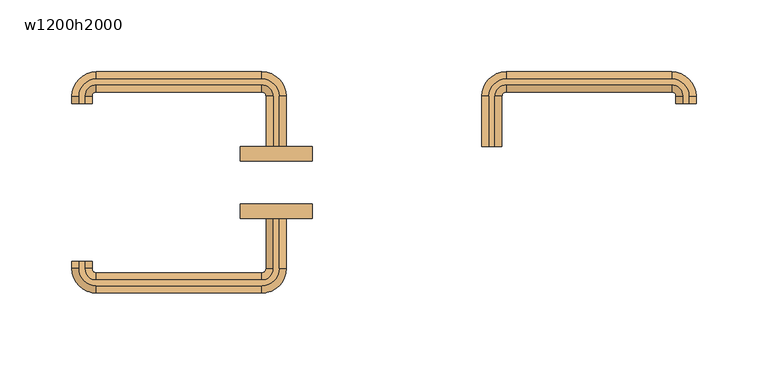
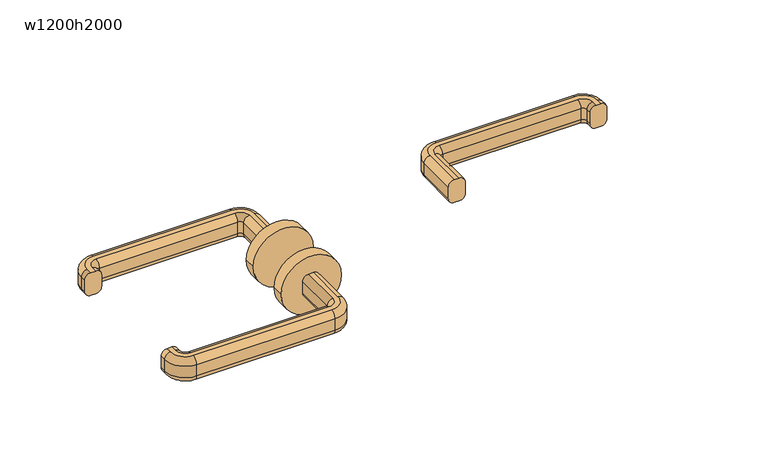
"""IFC4 building model written with IfcOpenShell, lengths in millimetres: door geometry, 二重 : w1200h2000."""

from ifc_helpers import new_model, si_unit, point, frame, frame_2d, origin, place, context, project, spatial, polyline, circle_curve, ellipse_curve, trimmed, segment, composite_curve, outline, extrude, source, transform, mapped, element, save
from ifc_brep_helpers import plane_surface, cylinder_surface, revolved_surface, advanced_brep


def w1200h2000_1489ebb8(model_context):
    return source(origin(), model_context, "Body", "SolidModel", [
        advanced_brep(
        [(-73.0, 95.0, 960.0), (-77.0, 95.0, 960.0), (-82.0, 95.0, 955.0), (-82.0, 95.0, 945.0477623), (-77.0, 95.0, 940.0477623), (-73.0, 95.0, 940.0477623), (-68.0, 95.0, 945.0477623), (-68.0, 95.0, 955.0), (-68.0, 130.0, 955.0), (-73.0, 130.0, 960.0), (-68.0, 130.0, 945.0477623), (-73.0, 130.0, 940.0477623), (-77.0, 130.0, 940.0477623), (-85.0, 138.0, 940.0477623), (-200.0, 138.0, 940.0477623), (-208.0, 130.0, 940.0477623), (-208.0, 125.0, 940.0477623), (-212.0, 125.0, 940.0477623), (-212.0, 130.0, 940.0477623), (-200.0, 142.0, 940.0477623), (-85.0, 142.0, 940.0477623), (-82.0, 130.0, 945.0477623), (-82.0, 130.0, 955.0), (-77.0, 130.0, 960.0), (-85.0, 142.0, 960.0), (-200.0, 142.0, 960.0), (-212.0, 130.0, 960.0), (-212.0, 125.0, 960.0), (-208.0, 125.0, 960.0), (-208.0, 130.0, 960.0), (-200.0, 138.0, 960.0), (-85.0, 138.0, 960.0), (-85.0, 147.0, 955.0), (-85.0, 147.0, 945.0477623), (-85.0, 133.0, 945.0477623), (-85.0, 133.0, 955.0), (-200.0, 147.0, 955.0), (-200.0, 147.0, 945.0477623), (-200.0, 133.0, 945.0477623), (-200.0, 133.0, 955.0), (-217.0, 130.0, 955.0), (-217.0, 130.0, 945.0477623), (-203.0, 130.0, 945.0477623), (-203.0, 130.0, 955.0), (-217.0, 125.0, 955.0), (-217.0, 125.0, 945.0477623), (-203.0, 125.0, 945.0477623), (-203.0, 125.0, 955.0)],
        [
            (0, 1),
            (1, 2, circle_curve(frame((-77.0, 95.0, 955.0), z_axis=(0.0, -1.0, 0.0), x_axis=(1.0, 0.0, 0.0)), 5.0)),
            (2, 3),
            (3, 4, circle_curve(frame((-77.0, 95.0, 945.0477623), z_axis=(0.0, -1.0, 0.0), x_axis=(1.0, 0.0, 0.0)), 5.0)),
            (4, 5),
            (5, 6, circle_curve(frame((-73.0, 95.0, 945.0477623), z_axis=(0.0, -1.0, 0.0), x_axis=(1.0, 0.0, 0.0)), 5.0)),
            (6, 7),
            (7, 0, circle_curve(frame((-73.0, 95.0, 955.0), z_axis=(0.0, -1.0, 0.0), x_axis=(1.0, 0.0, 0.0)), 5.0)),
            (7, 8),
            (8, 9, circle_curve(frame((-73.0, 130.0, 955.0), z_axis=(0.0, -1.0, 0.0), x_axis=(1.0, 0.0, 0.0)), 5.0)),
            (9, 0),
            (6, 10),
            (10, 8),
            (5, 11),
            (11, 10, circle_curve(frame((-73.0, 130.0, 945.0477623), z_axis=(0.0, -1.0, 0.0), x_axis=(1.0, 0.0, 0.0)), 5.0)),
            (4, 12),
            (12, 13, circle_curve(frame((-85.0, 130.0, 940.0477623), z_axis=(0.0, 0.0, 1.0), x_axis=(1.0, 0.0, 0.0)), 8.0)),
            (13, 14),
            (14, 15, circle_curve(frame((-200.0, 130.0, 940.0477623), z_axis=(0.0, 0.0, 1.0), x_axis=(0.0, 1.0, 0.0)), 8.0)),
            (15, 16),
            (16, 17),
            (17, 18),
            (18, 19, circle_curve(frame((-200.0, 130.0, 940.0477623), z_axis=(0.0, 0.0, -1.0), x_axis=(0.0, 1.0, 0.0)), 12.0)),
            (19, 20),
            (20, 11, circle_curve(frame((-85.0, 130.0, 940.0477623), z_axis=(0.0, 0.0, -1.0), x_axis=(1.0, 0.0, 0.0)), 12.0)),
            (3, 21),
            (21, 12, circle_curve(frame((-77.0, 130.0, 945.0477623), z_axis=(0.0, -1.0, 0.0), x_axis=(1.0, 0.0, 0.0)), 5.0)),
            (2, 22),
            (22, 21),
            (1, 23),
            (23, 22, circle_curve(frame((-77.0, 130.0, 955.0), z_axis=(0.0, -1.0, 0.0), x_axis=(1.0, 0.0, 0.0)), 5.0)),
            (9, 24, circle_curve(frame((-85.0, 130.0, 960.0), z_axis=(0.0, 0.0, 1.0), x_axis=(1.0, 0.0, 0.0)), 12.0)),
            (24, 25),
            (25, 26, circle_curve(frame((-200.0, 130.0, 960.0), z_axis=(0.0, 0.0, 1.0), x_axis=(0.0, 1.0, 0.0)), 12.0)),
            (26, 27),
            (27, 28),
            (28, 29),
            (29, 30, circle_curve(frame((-200.0, 130.0, 960.0), z_axis=(0.0, 0.0, -1.0), x_axis=(0.0, 1.0, 0.0)), 8.0)),
            (30, 31),
            (31, 23, circle_curve(frame((-85.0, 130.0, 960.0), z_axis=(0.0, 0.0, -1.0), x_axis=(1.0, 0.0, 0.0)), 8.0)),
            (32, 24, circle_curve(frame((-85.0, 142.0, 955.0), z_axis=(1.0, 0.0, 0.0), x_axis=(0.0, 1.0, 0.0)), 5.0)),
            (8, 32, circle_curve(frame((-85.0, 130.0, 955.0), z_axis=(0.0, 0.0, 1.0), x_axis=(1.0, 0.0, 0.0)), 17.0)),
            (33, 32),
            (10, 33, circle_curve(frame((-85.0, 130.0, 945.0477623), z_axis=(0.0, 0.0, 1.0), x_axis=(1.0, 0.0, 0.0)), 17.0)),
            (20, 33, circle_curve(frame((-85.0, 142.0, 945.0477623), z_axis=(1.0, 0.0, 0.0), x_axis=(0.0, 1.0, 0.0)), 5.0)),
            (34, 13, circle_curve(frame((-85.0, 138.0, 945.0477623), z_axis=(1.0, 0.0, 0.0), x_axis=(0.0, 1.0, 0.0)), 5.0)),
            (21, 34, circle_curve(frame((-85.0, 130.0, 945.0477623), z_axis=(0.0, 0.0, 1.0), x_axis=(1.0, 0.0, 0.0)), 3.0)),
            (35, 34),
            (22, 35, circle_curve(frame((-85.0, 130.0, 955.0), z_axis=(0.0, 0.0, 1.0), x_axis=(1.0, 0.0, 0.0)), 3.0)),
            (31, 35, circle_curve(frame((-85.0, 138.0, 955.0), z_axis=(1.0, 0.0, 0.0), x_axis=(0.0, 1.0, 0.0)), 5.0)),
            (32, 36),
            (36, 25, circle_curve(frame((-200.0, 142.0, 955.0), z_axis=(1.0, 0.0, 0.0), x_axis=(0.0, 1.0, 0.0)), 5.0)),
            (33, 37),
            (37, 36),
            (19, 37, circle_curve(frame((-200.0, 142.0, 945.0477623), z_axis=(1.0, 0.0, 0.0), x_axis=(0.0, 1.0, 0.0)), 5.0)),
            (34, 38),
            (38, 14, circle_curve(frame((-200.0, 138.0, 945.0477623), z_axis=(1.0, 0.0, 0.0), x_axis=(0.0, 1.0, 0.0)), 5.0)),
            (35, 39),
            (39, 38),
            (30, 39, circle_curve(frame((-200.0, 138.0, 955.0), z_axis=(1.0, 0.0, 0.0), x_axis=(0.0, 1.0, 0.0)), 5.0)),
            (40, 26, circle_curve(frame((-212.0, 130.0, 955.0), z_axis=(0.0, 1.0, 0.0), x_axis=(-1.0, 0.0, 0.0)), 5.0)),
            (36, 40, circle_curve(frame((-200.0, 130.0, 955.0), z_axis=(0.0, 0.0, 1.0), x_axis=(0.0, 1.0, 0.0)), 17.0)),
            (41, 40),
            (37, 41, circle_curve(frame((-200.0, 130.0, 945.0477623), z_axis=(0.0, 0.0, 1.0), x_axis=(0.0, 1.0, 0.0)), 17.0)),
            (18, 41, circle_curve(frame((-212.0, 130.0, 945.0477623), z_axis=(0.0, 1.0, 0.0), x_axis=(-1.0, 0.0, 0.0)), 5.0)),
            (42, 15, circle_curve(frame((-208.0, 130.0, 945.0477623), z_axis=(0.0, 1.0, 0.0), x_axis=(-1.0, 0.0, 0.0)), 5.0)),
            (38, 42, circle_curve(frame((-200.0, 130.0, 945.0477623), z_axis=(0.0, 0.0, 1.0), x_axis=(0.0, 1.0, 0.0)), 3.0)),
            (43, 42),
            (39, 43, circle_curve(frame((-200.0, 130.0, 955.0), z_axis=(0.0, 0.0, 1.0), x_axis=(0.0, 1.0, 0.0)), 3.0)),
            (29, 43, circle_curve(frame((-208.0, 130.0, 955.0), z_axis=(0.0, 1.0, 0.0), x_axis=(-1.0, 0.0, 0.0)), 5.0)),
            (27, 44, circle_curve(frame((-212.0, 125.0, 955.0), z_axis=(0.0, -1.0, 0.0), x_axis=(-1.0, 0.0, 0.0)), 5.0)),
            (44, 45),
            (45, 17, circle_curve(frame((-212.0, 125.0, 945.0477623), z_axis=(0.0, -1.0, 0.0), x_axis=(-1.0, 0.0, 0.0)), 5.0)),
            (16, 46, circle_curve(frame((-208.0, 125.0, 945.0477623), z_axis=(0.0, -1.0, 0.0), x_axis=(-1.0, 0.0, 0.0)), 5.0)),
            (46, 47),
            (47, 28, circle_curve(frame((-208.0, 125.0, 955.0), z_axis=(0.0, -1.0, 0.0), x_axis=(-1.0, 0.0, 0.0)), 5.0)),
            (40, 44),
            (41, 45),
            (42, 46),
            (43, 47),
        ],
        [
            plane_surface(frame((-64.801961, 95.0, 950.0), z_axis=(0.0, -1.0, 0.0), x_axis=(0.0, 0.0, 1.0))),
            cylinder_surface(frame((-73.0, 95.0, 955.0), z_axis=(0.0, -1.0, 0.0), x_axis=(1.0, 0.0, 0.0)), 5.0),
            plane_surface(frame((-68.0, 95.0, 955.0), z_axis=(1.0, 0.0, 0.0), x_axis=(0.0, 1.0, 0.0))),
            cylinder_surface(frame((-73.0, 95.0, 945.0477623), z_axis=(0.0, -1.0, 0.0), x_axis=(1.0, 0.0, 0.0)), 5.0),
            plane_surface(frame((-73.0, 95.0, 940.0477623), z_axis=(0.0, 0.0, -1.0), x_axis=(0.0, 1.0, 0.0))),
            cylinder_surface(frame((-77.0, 95.0, 945.0477623), z_axis=(0.0, -1.0, 0.0), x_axis=(1.0, 0.0, 0.0)), 5.0),
            plane_surface(frame((-82.0, 95.0, 945.0477623), z_axis=(-1.0, 0.0, 0.0), x_axis=(0.0, 1.0, 0.0))),
            cylinder_surface(frame((-77.0, 95.0, 955.0), z_axis=(0.0, -1.0, 0.0), x_axis=(1.0, 0.0, 0.0)), 5.0),
            plane_surface(frame((-77.0, 95.0, 960.0), z_axis=(0.0, 0.0, 1.0), x_axis=(0.0, 1.0, 0.0))),
            revolved_surface(trimmed(ellipse_curve(frame((-73.0, 130.0, 955.0), z_axis=(0.0, 1.0, 0.0), x_axis=(1.0, 0.0, 0.0)), 5.0, 5.0), [point((-73.0, 130.0, 960.0))], [point((-68.0, 130.0, 955.0))], True, "CARTESIAN"), (-85.0, 130.0, 950.0), (0.0, 0.0, -1.0)),
            cylinder_surface(frame((-85.0, 130.0, 950.0), z_axis=(0.0, 0.0, -1.0), x_axis=(1.0, 0.0, 0.0)), 17.0),
            revolved_surface(trimmed(ellipse_curve(frame((-73.0, 130.0, 945.0477623), z_axis=(0.0, 1.0, 0.0), x_axis=(1.0, 0.0, 0.0)), 5.0, 5.0), [point((-68.0, 130.0, 945.0477623))], [point((-73.0, 130.0, 940.0477623))], True, "CARTESIAN"), (-85.0, 130.0, 950.0), (0.0, 0.0, -1.0)),
            revolved_surface(trimmed(ellipse_curve(frame((-77.0, 130.0, 945.0477623), z_axis=(0.0, 1.0, 0.0), x_axis=(1.0, 0.0, 0.0)), 5.0, 5.0), [point((-77.0, 130.0, 940.0477623))], [point((-82.0, 130.0, 945.0477623))], True, "CARTESIAN"), (-85.0, 130.0, 950.0), (0.0, 0.0, -1.0)),
            revolved_surface(polyline([(-82.0, 130.0, 945.0477623), (-82.0, 130.0, 955.0)]), (-85.0, 130.0, 950.0), (0.0, 0.0, -1.0)),
            revolved_surface(trimmed(ellipse_curve(frame((-77.0, 130.0, 955.0), z_axis=(0.0, 1.0, 0.0), x_axis=(1.0, 0.0, 0.0)), 5.0, 5.0), [point((-82.0, 130.0, 955.0))], [point((-77.0, 130.0, 960.0))], True, "CARTESIAN"), (-85.0, 130.0, 950.0), (0.0, 0.0, -1.0)),
            cylinder_surface(frame((-85.0, 142.0, 955.0), z_axis=(1.0, 0.0, 0.0), x_axis=(0.0, 1.0, 0.0)), 5.0),
            plane_surface(frame((-85.0, 147.0, 955.0), z_axis=(0.0, 1.0, 0.0), x_axis=(-1.0, 0.0, 0.0))),
            cylinder_surface(frame((-85.0, 142.0, 945.0477623), z_axis=(1.0, 0.0, 0.0), x_axis=(0.0, 1.0, 0.0)), 5.0),
            cylinder_surface(frame((-85.0, 138.0, 945.0477623), z_axis=(1.0, 0.0, 0.0), x_axis=(0.0, 1.0, 0.0)), 5.0),
            plane_surface(frame((-85.0, 133.0, 945.0477623), z_axis=(0.0, -1.0, 0.0), x_axis=(-1.0, 0.0, 0.0))),
            cylinder_surface(frame((-85.0, 138.0, 955.0), z_axis=(1.0, 0.0, 0.0), x_axis=(0.0, 1.0, 0.0)), 5.0),
            revolved_surface(trimmed(ellipse_curve(frame((-200.0, 142.0, 955.0), z_axis=(-1.0, 0.0, 0.0), x_axis=(0.0, 1.0, 0.0)), 5.0, 5.0), [point((-200.0, 142.0, 960.0))], [point((-200.0, 147.0, 955.0))], True, "CARTESIAN"), (-200.0, 130.0, 950.0), (0.0, 0.0, -1.0)),
            cylinder_surface(frame((-200.0, 130.0, 950.0), z_axis=(0.0, 0.0, -1.0), x_axis=(0.0, 1.0, 0.0)), 17.0),
            revolved_surface(trimmed(ellipse_curve(frame((-200.0, 142.0, 945.0477623), z_axis=(-1.0, 0.0, 0.0), x_axis=(0.0, 1.0, 0.0)), 5.0, 5.0), [point((-200.0, 147.0, 945.0477623))], [point((-200.0, 142.0, 940.0477623))], True, "CARTESIAN"), (-200.0, 130.0, 950.0), (0.0, 0.0, -1.0)),
            revolved_surface(trimmed(ellipse_curve(frame((-200.0, 138.0, 945.0477623), z_axis=(-1.0, 0.0, 0.0), x_axis=(0.0, 1.0, 0.0)), 5.0, 5.0), [point((-200.0, 138.0, 940.0477623))], [point((-200.0, 133.0, 945.0477623))], True, "CARTESIAN"), (-200.0, 130.0, 950.0), (0.0, 0.0, -1.0)),
            revolved_surface(polyline([(-200.0, 133.0, 945.0477623), (-200.0, 133.0, 955.0)]), (-200.0, 130.0, 950.0), (0.0, 0.0, -1.0)),
            revolved_surface(trimmed(ellipse_curve(frame((-200.0, 138.0, 955.0), z_axis=(-1.0, 0.0, 0.0), x_axis=(0.0, 1.0, 0.0)), 5.0, 5.0), [point((-200.0, 133.0, 955.0))], [point((-200.0, 138.0, 960.0))], True, "CARTESIAN"), (-200.0, 130.0, 950.0), (0.0, 0.0, -1.0)),
            plane_surface(frame((-199.801961, 125.0, 950.0), z_axis=(0.0, -1.0, 0.0), x_axis=(0.0, 0.0, -1.0))),
            cylinder_surface(frame((-212.0, 130.0, 955.0), z_axis=(0.0, 1.0, 0.0), x_axis=(-1.0, 0.0, 0.0)), 5.0),
            plane_surface(frame((-217.0, 130.0, 955.0), z_axis=(-1.0, 0.0, 0.0), x_axis=(0.0, -1.0, 0.0))),
            cylinder_surface(frame((-212.0, 130.0, 945.0477623), z_axis=(0.0, 1.0, 0.0), x_axis=(-1.0, 0.0, 0.0)), 5.0),
            cylinder_surface(frame((-208.0, 130.0, 945.0477623), z_axis=(0.0, 1.0, 0.0), x_axis=(-1.0, 0.0, 0.0)), 5.0),
            plane_surface(frame((-203.0, 130.0, 945.0477623), z_axis=(1.0, 0.0, 0.0), x_axis=(0.0, -1.0, 0.0))),
            cylinder_surface(frame((-208.0, 130.0, 955.0), z_axis=(0.0, 1.0, 0.0), x_axis=(-1.0, 0.0, 0.0)), 5.0),
        ],
        [
            (0, [[1, 2, 3, 4, 5, 6, 7, 8]]),
            (1, [[9, 10, 11, -8]]),
            (2, [[12, 13, -9, -7]]),
            (3, [[14, 15, -12, -6]]),
            (4, [[16, 17, 18, 19, 20, 21, 22, 23, 24, 25, -14, -5]]),
            (5, [[26, 27, -16, -4]]),
            (6, [[28, 29, -26, -3]]),
            (7, [[30, 31, -28, -2]]),
            (8, [[-11, 32, 33, 34, 35, 36, 37, 38, 39, 40, -30, -1]]),
            (9, [[41, -32, -10, 42]]),
            (10, [[43, -42, -13, 44]]),
            (11, [[45, -44, -15, -25]]),
            (12, [[46, -17, -27, 47]]),
            (13, [[48, -47, -29, 49]]),
            (14, [[50, -49, -31, -40]]),
            (15, [[51, 52, -33, -41]]),
            (16, [[53, 54, -51, -43]]),
            (17, [[-24, 55, -53, -45]]),
            (18, [[56, 57, -18, -46]]),
            (19, [[58, 59, -56, -48]]),
            (20, [[-39, 60, -58, -50]]),
            (21, [[61, -34, -52, 62]]),
            (22, [[63, -62, -54, 64]]),
            (23, [[65, -64, -55, -23]]),
            (24, [[66, -19, -57, 67]]),
            (25, [[68, -67, -59, 69]]),
            (26, [[70, -69, -60, -38]]),
            (27, [[71, 72, 73, -21, 74, 75, 76, -36]]),
            (28, [[77, -71, -35, -61]]),
            (29, [[78, -72, -77, -63]]),
            (30, [[-22, -73, -78, -65]]),
            (31, [[79, -74, -20, -66]]),
            (32, [[80, -75, -79, -68]]),
            (33, [[-37, -76, -80, -70]]),
        ],
    ),
        advanced_brep(
        [(-77.0, 45.0, 940.0), (-82.0, 45.0, 945.0), (-82.0, 45.0, 955.0), (-77.0, 45.0, 960.0), (-73.0, 45.0, 960.0), (-68.0, 45.0, 955.0), (-68.0, 45.0, 945.0), (-73.0, 45.0, 940.0), (-73.0, 10.0, 940.0), (-85.0, -2.0, 940.0), (-200.0, -2.0, 940.0), (-212.0, 10.0, 940.0), (-212.0, 15.0, 940.0), (-208.0, 15.0, 940.0), (-208.0, 10.0, 940.0), (-200.0, 2.0, 940.0), (-85.0, 2.0, 940.0), (-77.0, 10.0, 940.0), (-68.0, 10.0, 945.0), (-68.0, 10.0, 955.0), (-73.0, 10.0, 960.0), (-77.0, 10.0, 960.0), (-85.0, 2.0, 960.0), (-200.0, 2.0, 960.0), (-208.0, 10.0, 960.0), (-208.0, 15.0, 960.0), (-212.0, 15.0, 960.0), (-212.0, 10.0, 960.0), (-200.0, -2.0, 960.0), (-85.0, -2.0, 960.0), (-82.0, 10.0, 955.0), (-82.0, 10.0, 945.0), (-85.0, -7.0, 945.0), (-85.0, -7.0, 955.0), (-85.0, 7.0, 955.0), (-85.0, 7.0, 945.0), (-200.0, -7.0, 945.0), (-200.0, -7.0, 955.0), (-200.0, 7.0, 955.0), (-200.0, 7.0, 945.0), (-217.0, 10.0, 945.0), (-217.0, 10.0, 955.0), (-203.0, 10.0, 955.0), (-203.0, 10.0, 945.0), (-217.0, 15.0, 945.0), (-217.0, 15.0, 955.0), (-203.0, 15.0, 955.0), (-203.0, 15.0, 945.0)],
        [
            (0, 1, circle_curve(frame((-77.0, 45.0, 945.0), z_axis=(0.0, 1.0, 0.0), x_axis=(-1.0, 0.0, 0.0)), 5.0)),
            (1, 2),
            (2, 3, circle_curve(frame((-77.0, 45.0, 955.0), z_axis=(0.0, 1.0, 0.0), x_axis=(-1.0, 0.0, 0.0)), 5.0)),
            (3, 4),
            (4, 5, circle_curve(frame((-73.0, 45.0, 955.0), z_axis=(0.0, 1.0, 0.0), x_axis=(-1.0, 0.0, 0.0)), 5.0)),
            (5, 6),
            (6, 7, circle_curve(frame((-73.0, 45.0, 945.0), z_axis=(0.0, 1.0, 0.0), x_axis=(-1.0, 0.0, 0.0)), 5.0)),
            (7, 0),
            (7, 8),
            (8, 9, circle_curve(frame((-85.0, 10.0, 940.0), z_axis=(0.0, 0.0, -1.0), x_axis=(1.0, 0.0, 0.0)), 12.0)),
            (9, 10),
            (10, 11, circle_curve(frame((-200.0, 10.0, 940.0), z_axis=(0.0, 0.0, -1.0), x_axis=(0.0, -1.0, 0.0)), 12.0)),
            (11, 12),
            (12, 13),
            (13, 14),
            (14, 15, circle_curve(frame((-200.0, 10.0, 940.0), z_axis=(0.0, 0.0, 1.0), x_axis=(0.0, -1.0, 0.0)), 8.0)),
            (15, 16),
            (16, 17, circle_curve(frame((-85.0, 10.0, 940.0), z_axis=(0.0, 0.0, 1.0), x_axis=(1.0, 0.0, 0.0)), 8.0)),
            (17, 0),
            (6, 18),
            (18, 8, circle_curve(frame((-73.0, 10.0, 945.0), z_axis=(0.0, 1.0, 0.0), x_axis=(-1.0, 0.0, 0.0)), 5.0)),
            (5, 19),
            (19, 18),
            (4, 20),
            (20, 19, circle_curve(frame((-73.0, 10.0, 955.0), z_axis=(0.0, 1.0, 0.0), x_axis=(-1.0, 0.0, 0.0)), 5.0)),
            (3, 21),
            (21, 22, circle_curve(frame((-85.0, 10.0, 960.0), z_axis=(0.0, 0.0, -1.0), x_axis=(1.0, 0.0, 0.0)), 8.0)),
            (22, 23),
            (23, 24, circle_curve(frame((-200.0, 10.0, 960.0), z_axis=(0.0, 0.0, -1.0), x_axis=(0.0, -1.0, 0.0)), 8.0)),
            (24, 25),
            (25, 26),
            (26, 27),
            (27, 28, circle_curve(frame((-200.0, 10.0, 960.0), z_axis=(0.0, 0.0, 1.0), x_axis=(0.0, -1.0, 0.0)), 12.0)),
            (28, 29),
            (29, 20, circle_curve(frame((-85.0, 10.0, 960.0), z_axis=(0.0, 0.0, 1.0), x_axis=(1.0, 0.0, 0.0)), 12.0)),
            (2, 30),
            (30, 21, circle_curve(frame((-77.0, 10.0, 955.0), z_axis=(0.0, 1.0, 0.0), x_axis=(-1.0, 0.0, 0.0)), 5.0)),
            (1, 31),
            (31, 30),
            (17, 31, circle_curve(frame((-77.0, 10.0, 945.0), z_axis=(0.0, 1.0, 0.0), x_axis=(-1.0, 0.0, 0.0)), 5.0)),
            (32, 9, circle_curve(frame((-85.0, -2.0, 945.0), z_axis=(1.0, 0.0, 0.0), x_axis=(0.0, 1.0, 0.0)), 5.0)),
            (18, 32, circle_curve(frame((-85.0, 10.0, 945.0), z_axis=(0.0, 0.0, -1.0), x_axis=(1.0, 0.0, 0.0)), 17.0)),
            (33, 32),
            (19, 33, circle_curve(frame((-85.0, 10.0, 955.0), z_axis=(0.0, 0.0, -1.0), x_axis=(1.0, 0.0, 0.0)), 17.0)),
            (29, 33, circle_curve(frame((-85.0, -2.0, 955.0), z_axis=(1.0, 0.0, 0.0), x_axis=(0.0, 1.0, 0.0)), 5.0)),
            (34, 22, circle_curve(frame((-85.0, 2.0, 955.0), z_axis=(1.0, 0.0, 0.0), x_axis=(0.0, 1.0, 0.0)), 5.0)),
            (30, 34, circle_curve(frame((-85.0, 10.0, 955.0), z_axis=(0.0, 0.0, -1.0), x_axis=(1.0, 0.0, 0.0)), 3.0)),
            (35, 34),
            (31, 35, circle_curve(frame((-85.0, 10.0, 945.0), z_axis=(0.0, 0.0, -1.0), x_axis=(1.0, 0.0, 0.0)), 3.0)),
            (16, 35, circle_curve(frame((-85.0, 2.0, 945.0), z_axis=(1.0, 0.0, 0.0), x_axis=(0.0, 1.0, 0.0)), 5.0)),
            (32, 36),
            (36, 10, circle_curve(frame((-200.0, -2.0, 945.0), z_axis=(1.0, 0.0, 0.0), x_axis=(0.0, 1.0, 0.0)), 5.0)),
            (33, 37),
            (37, 36),
            (28, 37, circle_curve(frame((-200.0, -2.0, 955.0), z_axis=(1.0, 0.0, 0.0), x_axis=(0.0, 1.0, 0.0)), 5.0)),
            (34, 38),
            (38, 23, circle_curve(frame((-200.0, 2.0, 955.0), z_axis=(1.0, 0.0, 0.0), x_axis=(0.0, 1.0, 0.0)), 5.0)),
            (35, 39),
            (39, 38),
            (15, 39, circle_curve(frame((-200.0, 2.0, 945.0), z_axis=(1.0, 0.0, 0.0), x_axis=(0.0, 1.0, 0.0)), 5.0)),
            (40, 11, circle_curve(frame((-212.0, 10.0, 945.0), z_axis=(0.0, -1.0, 0.0), x_axis=(1.0, 0.0, 0.0)), 5.0)),
            (36, 40, circle_curve(frame((-200.0, 10.0, 945.0), z_axis=(0.0, 0.0, -1.0), x_axis=(0.0, -1.0, 0.0)), 17.0)),
            (41, 40),
            (37, 41, circle_curve(frame((-200.0, 10.0, 955.0), z_axis=(0.0, 0.0, -1.0), x_axis=(0.0, -1.0, 0.0)), 17.0)),
            (27, 41, circle_curve(frame((-212.0, 10.0, 955.0), z_axis=(0.0, -1.0, 0.0), x_axis=(1.0, 0.0, 0.0)), 5.0)),
            (42, 24, circle_curve(frame((-208.0, 10.0, 955.0), z_axis=(0.0, -1.0, 0.0), x_axis=(1.0, 0.0, 0.0)), 5.0)),
            (38, 42, circle_curve(frame((-200.0, 10.0, 955.0), z_axis=(0.0, 0.0, -1.0), x_axis=(0.0, -1.0, 0.0)), 3.0)),
            (43, 42),
            (39, 43, circle_curve(frame((-200.0, 10.0, 945.0), z_axis=(0.0, 0.0, -1.0), x_axis=(0.0, -1.0, 0.0)), 3.0)),
            (14, 43, circle_curve(frame((-208.0, 10.0, 945.0), z_axis=(0.0, -1.0, 0.0), x_axis=(1.0, 0.0, 0.0)), 5.0)),
            (12, 44, circle_curve(frame((-212.0, 15.0, 945.0), z_axis=(0.0, 1.0, 0.0), x_axis=(1.0, 0.0, 0.0)), 5.0)),
            (44, 45),
            (45, 26, circle_curve(frame((-212.0, 15.0, 955.0), z_axis=(0.0, 1.0, 0.0), x_axis=(1.0, 0.0, 0.0)), 5.0)),
            (25, 46, circle_curve(frame((-208.0, 15.0, 955.0), z_axis=(0.0, 1.0, 0.0), x_axis=(1.0, 0.0, 0.0)), 5.0)),
            (46, 47),
            (47, 13, circle_curve(frame((-208.0, 15.0, 945.0), z_axis=(0.0, 1.0, 0.0), x_axis=(1.0, 0.0, 0.0)), 5.0)),
            (40, 44),
            (41, 45),
            (42, 46),
            (43, 47),
        ],
        [
            plane_surface(frame((-64.801961, 45.0, 950.0), z_axis=(0.0, 1.0, 0.0), x_axis=(0.0, 0.0, -1.0))),
            plane_surface(frame((-77.0, 45.0, 940.0), z_axis=(0.0, 0.0, -1.0), x_axis=(0.0, -1.0, 0.0))),
            cylinder_surface(frame((-73.0, 45.0, 945.0), z_axis=(0.0, 1.0, 0.0), x_axis=(-1.0, 0.0, 0.0)), 5.0),
            plane_surface(frame((-68.0, 45.0, 945.0), z_axis=(1.0, 0.0, 0.0), x_axis=(0.0, -1.0, 0.0))),
            cylinder_surface(frame((-73.0, 45.0, 955.0), z_axis=(0.0, 1.0, 0.0), x_axis=(-1.0, 0.0, 0.0)), 5.0),
            plane_surface(frame((-73.0, 45.0, 960.0), z_axis=(0.0, 0.0, 1.0), x_axis=(0.0, -1.0, 0.0))),
            cylinder_surface(frame((-77.0, 45.0, 955.0), z_axis=(0.0, 1.0, 0.0), x_axis=(-1.0, 0.0, 0.0)), 5.0),
            plane_surface(frame((-82.0, 45.0, 955.0), z_axis=(-1.0, 0.0, 0.0), x_axis=(0.0, -1.0, 0.0))),
            cylinder_surface(frame((-77.0, 45.0, 945.0), z_axis=(0.0, 1.0, 0.0), x_axis=(-1.0, 0.0, 0.0)), 5.0),
            revolved_surface(trimmed(ellipse_curve(frame((-73.0, 10.0, 945.0), z_axis=(0.0, -1.0, 0.0), x_axis=(-1.0, 0.0, 0.0)), 5.0, 5.0), [point((-73.0, 10.0, 940.0))], [point((-68.0, 10.0, 945.0))], True, "CARTESIAN"), (-85.0, 10.0, 950.0), (0.0, 0.0, 1.0)),
            cylinder_surface(frame((-85.0, 10.0, 950.0), z_axis=(0.0, 0.0, 1.0), x_axis=(1.0, 0.0, 0.0)), 17.0),
            revolved_surface(trimmed(ellipse_curve(frame((-73.0, 10.0, 955.0), z_axis=(0.0, -1.0, 0.0), x_axis=(-1.0, 0.0, 0.0)), 5.0, 5.0), [point((-68.0, 10.0, 955.0))], [point((-73.0, 10.0, 960.0))], True, "CARTESIAN"), (-85.0, 10.0, 950.0), (0.0, 0.0, 1.0)),
            revolved_surface(trimmed(ellipse_curve(frame((-77.0, 10.0, 955.0), z_axis=(0.0, -1.0, 0.0), x_axis=(-1.0, 0.0, 0.0)), 5.0, 5.0), [point((-77.0, 10.0, 960.0))], [point((-82.0, 10.0, 955.0))], True, "CARTESIAN"), (-85.0, 10.0, 950.0), (0.0, 0.0, 1.0)),
            revolved_surface(polyline([(-82.0, 10.0, 955.0), (-82.0, 10.0, 945.0)]), (-85.0, 10.0, 950.0), (0.0, 0.0, 1.0)),
            revolved_surface(trimmed(ellipse_curve(frame((-77.0, 10.0, 945.0), z_axis=(0.0, -1.0, 0.0), x_axis=(-1.0, 0.0, 0.0)), 5.0, 5.0), [point((-82.0, 10.0, 945.0))], [point((-77.0, 10.0, 940.0))], True, "CARTESIAN"), (-85.0, 10.0, 950.0), (0.0, 0.0, 1.0)),
            cylinder_surface(frame((-85.0, -2.0, 945.0), z_axis=(1.0, 0.0, 0.0), x_axis=(0.0, 1.0, 0.0)), 5.0),
            plane_surface(frame((-85.0, -7.0, 945.0), z_axis=(0.0, -1.0, 0.0), x_axis=(-1.0, 0.0, 0.0))),
            cylinder_surface(frame((-85.0, -2.0, 955.0), z_axis=(1.0, 0.0, 0.0), x_axis=(0.0, 1.0, 0.0)), 5.0),
            cylinder_surface(frame((-85.0, 2.0, 955.0), z_axis=(1.0, 0.0, 0.0), x_axis=(0.0, 1.0, 0.0)), 5.0),
            plane_surface(frame((-85.0, 7.0, 955.0), z_axis=(0.0, 1.0, 0.0), x_axis=(-1.0, 0.0, 0.0))),
            cylinder_surface(frame((-85.0, 2.0, 945.0), z_axis=(1.0, 0.0, 0.0), x_axis=(0.0, 1.0, 0.0)), 5.0),
            revolved_surface(trimmed(ellipse_curve(frame((-200.0, -2.0, 945.0), z_axis=(-1.0, 0.0, 0.0), x_axis=(0.0, 1.0, 0.0)), 5.0, 5.0), [point((-200.0, -2.0, 940.0))], [point((-200.0, -7.0, 945.0))], True, "CARTESIAN"), (-200.0, 10.0, 950.0), (0.0, 0.0, 1.0)),
            cylinder_surface(frame((-200.0, 10.0, 950.0), z_axis=(0.0, 0.0, 1.0), x_axis=(0.0, -1.0, 0.0)), 17.0),
            revolved_surface(trimmed(ellipse_curve(frame((-200.0, -2.0, 955.0), z_axis=(-1.0, 0.0, 0.0), x_axis=(0.0, 1.0, 0.0)), 5.0, 5.0), [point((-200.0, -7.0, 955.0))], [point((-200.0, -2.0, 960.0))], True, "CARTESIAN"), (-200.0, 10.0, 950.0), (0.0, 0.0, 1.0)),
            revolved_surface(trimmed(ellipse_curve(frame((-200.0, 2.0, 955.0), z_axis=(-1.0, 0.0, 0.0), x_axis=(0.0, 1.0, 0.0)), 5.0, 5.0), [point((-200.0, 2.0, 960.0))], [point((-200.0, 7.0, 955.0))], True, "CARTESIAN"), (-200.0, 10.0, 950.0), (0.0, 0.0, 1.0)),
            revolved_surface(polyline([(-200.0, 7.0, 955.0), (-200.0, 7.0, 945.0)]), (-200.0, 10.0, 950.0), (0.0, 0.0, 1.0)),
            revolved_surface(trimmed(ellipse_curve(frame((-200.0, 2.0, 945.0), z_axis=(-1.0, 0.0, 0.0), x_axis=(0.0, 1.0, 0.0)), 5.0, 5.0), [point((-200.0, 7.0, 945.0))], [point((-200.0, 2.0, 940.0))], True, "CARTESIAN"), (-200.0, 10.0, 950.0), (0.0, 0.0, 1.0)),
            plane_surface(frame((-199.801961, 15.0, 950.0), z_axis=(0.0, 1.0, 0.0), x_axis=(0.0, 0.0, 1.0))),
            cylinder_surface(frame((-212.0, 10.0, 945.0), z_axis=(0.0, -1.0, 0.0), x_axis=(1.0, 0.0, 0.0)), 5.0),
            plane_surface(frame((-217.0, 10.0, 945.0), z_axis=(-1.0, 0.0, 0.0), x_axis=(0.0, 1.0, 0.0))),
            cylinder_surface(frame((-212.0, 10.0, 955.0), z_axis=(0.0, -1.0, 0.0), x_axis=(1.0, 0.0, 0.0)), 5.0),
            cylinder_surface(frame((-208.0, 10.0, 955.0), z_axis=(0.0, -1.0, 0.0), x_axis=(1.0, 0.0, 0.0)), 5.0),
            plane_surface(frame((-203.0, 10.0, 955.0), z_axis=(1.0, 0.0, 0.0), x_axis=(0.0, 1.0, 0.0))),
            cylinder_surface(frame((-208.0, 10.0, 945.0), z_axis=(0.0, -1.0, 0.0), x_axis=(1.0, 0.0, 0.0)), 5.0),
        ],
        [
            (0, [[1, 2, 3, 4, 5, 6, 7, 8]]),
            (1, [[9, 10, 11, 12, 13, 14, 15, 16, 17, 18, 19, -8]]),
            (2, [[20, 21, -9, -7]]),
            (3, [[22, 23, -20, -6]]),
            (4, [[24, 25, -22, -5]]),
            (5, [[26, 27, 28, 29, 30, 31, 32, 33, 34, 35, -24, -4]]),
            (6, [[36, 37, -26, -3]]),
            (7, [[38, 39, -36, -2]]),
            (8, [[-19, 40, -38, -1]]),
            (9, [[41, -10, -21, 42]]),
            (10, [[43, -42, -23, 44]]),
            (11, [[45, -44, -25, -35]]),
            (12, [[46, -27, -37, 47]]),
            (13, [[48, -47, -39, 49]]),
            (14, [[50, -49, -40, -18]]),
            (15, [[51, 52, -11, -41]]),
            (16, [[53, 54, -51, -43]]),
            (17, [[-34, 55, -53, -45]]),
            (18, [[56, 57, -28, -46]]),
            (19, [[58, 59, -56, -48]]),
            (20, [[-17, 60, -58, -50]]),
            (21, [[61, -12, -52, 62]]),
            (22, [[63, -62, -54, 64]]),
            (23, [[65, -64, -55, -33]]),
            (24, [[66, -29, -57, 67]]),
            (25, [[68, -67, -59, 69]]),
            (26, [[70, -69, -60, -16]]),
            (27, [[-14, 71, 72, 73, -31, 74, 75, 76]]),
            (28, [[77, -71, -13, -61]]),
            (29, [[78, -72, -77, -63]]),
            (30, [[-32, -73, -78, -65]]),
            (31, [[79, -74, -30, -66]]),
            (32, [[80, -75, -79, -68]]),
            (33, [[-15, -76, -80, -70]]),
        ],
    ),
        extrude(outline(composite_curve([segment(trimmed(circle_curve(frame_2d((950.0, -75.0)), 25.0), [point((950.0, -50.0))], [point((950.0, -100.0))], False, "CARTESIAN"), True, "CONTINUOUS"), segment(trimmed(circle_curve(frame_2d((950.0, -75.0)), 25.0), [point((950.0, -100.0))], [point((950.0, -50.0))], False, "CARTESIAN"), True, "CONTINUOUS")], self_intersect=False)), frame((0.0, 85.0, 0.0), z_axis=(0.0, 1.0, 0.0), x_axis=(0.0, 0.0, 1.0)), (0.0, 0.0, 1.0), 10.0),
        extrude(outline(composite_curve([segment(trimmed(circle_curve(frame_2d((950.0, -75.0)), 25.0), [point((950.0, -50.0))], [point((950.0, -100.0))], False, "CARTESIAN"), True, "CONTINUOUS"), segment(trimmed(circle_curve(frame_2d((950.0, -75.0)), 25.0), [point((950.0, -100.0))], [point((950.0, -50.0))], False, "CARTESIAN"), True, "CONTINUOUS")], self_intersect=False)), frame((0.0, 45.0, 0.0), z_axis=(0.0, 1.0, 0.0), x_axis=(0.0, 0.0, 1.0)), (0.0, 0.0, 1.0), 10.0),
        advanced_brep(
        [(73.0, 95.0, 960.0), (68.0, 95.0, 955.0), (68.0, 95.0, 945.0477623), (73.0, 95.0, 940.0477623), (77.0, 95.0, 940.0477623), (82.0, 95.0, 945.0477623), (82.0, 95.0, 955.0), (77.0, 95.0, 960.0), (73.0, 130.0, 960.0), (68.0, 130.0, 955.0), (68.0, 130.0, 945.0477623), (73.0, 130.0, 940.0477623), (85.0, 142.0, 940.0477623), (200.0, 142.0, 940.0477623), (212.0, 130.0, 940.0477623), (212.0, 125.0, 940.0477623), (208.0, 125.0, 940.0477623), (208.0, 130.0, 940.0477623), (200.0, 138.0, 940.0477623), (85.0, 138.0, 940.0477623), (77.0, 130.0, 940.0477623), (82.0, 130.0, 945.0477623), (82.0, 130.0, 955.0), (77.0, 130.0, 960.0), (85.0, 138.0, 960.0), (200.0, 138.0, 960.0), (208.0, 130.0, 960.0), (208.0, 125.0, 960.0), (212.0, 125.0, 960.0), (212.0, 130.0, 960.0), (200.0, 142.0, 960.0), (85.0, 142.0, 960.0), (85.0, 147.0, 955.0), (85.0, 147.0, 945.0477623), (85.0, 133.0, 945.0477623), (85.0, 133.0, 955.0), (200.0, 147.0, 955.0), (200.0, 147.0, 945.0477623), (200.0, 133.0, 945.0477623), (200.0, 133.0, 955.0), (217.0, 130.0, 955.0), (217.0, 130.0, 945.0477623), (203.0, 130.0, 945.0477623), (203.0, 130.0, 955.0), (203.0, 125.0, 955.0), (203.0, 125.0, 945.0477623), (217.0, 125.0, 945.0477623), (217.0, 125.0, 955.0)],
        [
            (0, 1, circle_curve(frame((73.0, 95.0, 955.0), z_axis=(0.0, -1.0, 0.0), x_axis=(-1.0, 0.0, 0.0)), 5.0)),
            (1, 2),
            (2, 3, circle_curve(frame((73.0, 95.0, 945.0477623), z_axis=(0.0, -1.0, 0.0), x_axis=(-1.0, 0.0, 0.0)), 5.0)),
            (3, 4),
            (4, 5, circle_curve(frame((77.0, 95.0, 945.0477623), z_axis=(0.0, -1.0, 0.0), x_axis=(-1.0, 0.0, 0.0)), 5.0)),
            (5, 6),
            (6, 7, circle_curve(frame((77.0, 95.0, 955.0), z_axis=(0.0, -1.0, 0.0), x_axis=(-1.0, 0.0, 0.0)), 5.0)),
            (7, 0),
            (0, 8),
            (8, 9, circle_curve(frame((73.0, 130.0, 955.0), z_axis=(0.0, -1.0, 0.0), x_axis=(-1.0, 0.0, 0.0)), 5.0)),
            (9, 1),
            (9, 10),
            (10, 2),
            (10, 11, circle_curve(frame((73.0, 130.0, 945.0477623), z_axis=(0.0, -1.0, 0.0), x_axis=(-1.0, 0.0, 0.0)), 5.0)),
            (11, 3),
            (11, 12, circle_curve(frame((85.0, 130.0, 940.0477623), z_axis=(0.0, 0.0, -1.0), x_axis=(-1.0, 0.0, 0.0)), 12.0)),
            (12, 13),
            (13, 14, circle_curve(frame((200.0, 130.0, 940.0477623), z_axis=(0.0, 0.0, -1.0), x_axis=(0.0, 1.0, 0.0)), 12.0)),
            (14, 15),
            (15, 16),
            (16, 17),
            (17, 18, circle_curve(frame((200.0, 130.0, 940.0477623), z_axis=(0.0, 0.0, 1.0), x_axis=(0.0, 1.0, 0.0)), 8.0)),
            (18, 19),
            (19, 20, circle_curve(frame((85.0, 130.0, 940.0477623), z_axis=(0.0, 0.0, 1.0), x_axis=(-1.0, 0.0, 0.0)), 8.0)),
            (20, 4),
            (20, 21, circle_curve(frame((77.0, 130.0, 945.0477623), z_axis=(0.0, -1.0, 0.0), x_axis=(-1.0, 0.0, 0.0)), 5.0)),
            (21, 5),
            (21, 22),
            (22, 6),
            (22, 23, circle_curve(frame((77.0, 130.0, 955.0), z_axis=(0.0, -1.0, 0.0), x_axis=(-1.0, 0.0, 0.0)), 5.0)),
            (23, 7),
            (23, 24, circle_curve(frame((85.0, 130.0, 960.0), z_axis=(0.0, 0.0, -1.0), x_axis=(-1.0, 0.0, 0.0)), 8.0)),
            (24, 25),
            (25, 26, circle_curve(frame((200.0, 130.0, 960.0), z_axis=(0.0, 0.0, -1.0), x_axis=(0.0, 1.0, 0.0)), 8.0)),
            (26, 27),
            (27, 28),
            (28, 29),
            (29, 30, circle_curve(frame((200.0, 130.0, 960.0), z_axis=(0.0, 0.0, 1.0), x_axis=(0.0, 1.0, 0.0)), 12.0)),
            (30, 31),
            (31, 8, circle_curve(frame((85.0, 130.0, 960.0), z_axis=(0.0, 0.0, 1.0), x_axis=(-1.0, 0.0, 0.0)), 12.0)),
            (32, 9, circle_curve(frame((85.0, 130.0, 955.0), z_axis=(0.0, 0.0, 1.0), x_axis=(-1.0, 0.0, 0.0)), 17.0)),
            (31, 32, circle_curve(frame((85.0, 142.0, 955.0), z_axis=(-1.0, 0.0, 0.0), x_axis=(0.0, 1.0, 0.0)), 5.0)),
            (33, 10, circle_curve(frame((85.0, 130.0, 945.0477623), z_axis=(0.0, 0.0, 1.0), x_axis=(-1.0, 0.0, 0.0)), 17.0)),
            (32, 33),
            (33, 12, circle_curve(frame((85.0, 142.0, 945.0477623), z_axis=(-1.0, 0.0, 0.0), x_axis=(0.0, 1.0, 0.0)), 5.0)),
            (34, 21, circle_curve(frame((85.0, 130.0, 945.0477623), z_axis=(0.0, 0.0, 1.0), x_axis=(-1.0, 0.0, 0.0)), 3.0)),
            (19, 34, circle_curve(frame((85.0, 138.0, 945.0477623), z_axis=(-1.0, 0.0, 0.0), x_axis=(0.0, 1.0, 0.0)), 5.0)),
            (35, 22, circle_curve(frame((85.0, 130.0, 955.0), z_axis=(0.0, 0.0, 1.0), x_axis=(-1.0, 0.0, 0.0)), 3.0)),
            (34, 35),
            (35, 24, circle_curve(frame((85.0, 138.0, 955.0), z_axis=(-1.0, 0.0, 0.0), x_axis=(0.0, 1.0, 0.0)), 5.0)),
            (30, 36, circle_curve(frame((200.0, 142.0, 955.0), z_axis=(-1.0, 0.0, 0.0), x_axis=(0.0, 1.0, 0.0)), 5.0)),
            (36, 32),
            (36, 37),
            (37, 33),
            (37, 13, circle_curve(frame((200.0, 142.0, 945.0477623), z_axis=(-1.0, 0.0, 0.0), x_axis=(0.0, 1.0, 0.0)), 5.0)),
            (18, 38, circle_curve(frame((200.0, 138.0, 945.0477623), z_axis=(-1.0, 0.0, 0.0), x_axis=(0.0, 1.0, 0.0)), 5.0)),
            (38, 34),
            (38, 39),
            (39, 35),
            (39, 25, circle_curve(frame((200.0, 138.0, 955.0), z_axis=(-1.0, 0.0, 0.0), x_axis=(0.0, 1.0, 0.0)), 5.0)),
            (40, 36, circle_curve(frame((200.0, 130.0, 955.0), z_axis=(0.0, 0.0, 1.0), x_axis=(0.0, 1.0, 0.0)), 17.0)),
            (29, 40, circle_curve(frame((212.0, 130.0, 955.0), z_axis=(0.0, 1.0, 0.0), x_axis=(1.0, 0.0, 0.0)), 5.0)),
            (41, 37, circle_curve(frame((200.0, 130.0, 945.0477623), z_axis=(0.0, 0.0, 1.0), x_axis=(0.0, 1.0, 0.0)), 17.0)),
            (40, 41),
            (41, 14, circle_curve(frame((212.0, 130.0, 945.0477623), z_axis=(0.0, 1.0, 0.0), x_axis=(1.0, 0.0, 0.0)), 5.0)),
            (42, 38, circle_curve(frame((200.0, 130.0, 945.0477623), z_axis=(0.0, 0.0, 1.0), x_axis=(0.0, 1.0, 0.0)), 3.0)),
            (17, 42, circle_curve(frame((208.0, 130.0, 945.0477623), z_axis=(0.0, 1.0, 0.0), x_axis=(1.0, 0.0, 0.0)), 5.0)),
            (43, 39, circle_curve(frame((200.0, 130.0, 955.0), z_axis=(0.0, 0.0, 1.0), x_axis=(0.0, 1.0, 0.0)), 3.0)),
            (42, 43),
            (43, 26, circle_curve(frame((208.0, 130.0, 955.0), z_axis=(0.0, 1.0, 0.0), x_axis=(1.0, 0.0, 0.0)), 5.0)),
            (27, 44, circle_curve(frame((208.0, 125.0, 955.0), z_axis=(0.0, -1.0, 0.0), x_axis=(1.0, 0.0, 0.0)), 5.0)),
            (44, 45),
            (45, 16, circle_curve(frame((208.0, 125.0, 945.0477623), z_axis=(0.0, -1.0, 0.0), x_axis=(1.0, 0.0, 0.0)), 5.0)),
            (15, 46, circle_curve(frame((212.0, 125.0, 945.0477623), z_axis=(0.0, -1.0, 0.0), x_axis=(1.0, 0.0, 0.0)), 5.0)),
            (46, 47),
            (47, 28, circle_curve(frame((212.0, 125.0, 955.0), z_axis=(0.0, -1.0, 0.0), x_axis=(1.0, 0.0, 0.0)), 5.0)),
            (47, 40),
            (46, 41),
            (45, 42),
            (44, 43),
        ],
        [
            plane_surface(frame((64.801961, 95.0, 950.0), z_axis=(0.0, -1.0, 0.0), x_axis=(0.0, 0.0, 1.0))),
            cylinder_surface(frame((73.0, 95.0, 955.0), z_axis=(0.0, -1.0, 0.0), x_axis=(-1.0, 0.0, 0.0)), 5.0),
            plane_surface(frame((68.0, 95.0, 955.0), z_axis=(-1.0, 0.0, 0.0), x_axis=(0.0, 1.0, 0.0))),
            cylinder_surface(frame((73.0, 95.0, 945.0477623), z_axis=(0.0, -1.0, 0.0), x_axis=(-1.0, 0.0, 0.0)), 5.0),
            plane_surface(frame((73.0, 95.0, 940.0477623), z_axis=(0.0, 0.0, -1.0), x_axis=(0.0, 1.0, 0.0))),
            cylinder_surface(frame((77.0, 95.0, 945.0477623), z_axis=(0.0, -1.0, 0.0), x_axis=(-1.0, 0.0, 0.0)), 5.0),
            plane_surface(frame((82.0, 95.0, 945.0477623), z_axis=(1.0, 0.0, 0.0), x_axis=(0.0, 1.0, 0.0))),
            cylinder_surface(frame((77.0, 95.0, 955.0), z_axis=(0.0, -1.0, 0.0), x_axis=(-1.0, 0.0, 0.0)), 5.0),
            plane_surface(frame((77.0, 95.0, 960.0), z_axis=(0.0, 0.0, 1.0), x_axis=(0.0, 1.0, 0.0))),
            revolved_surface(trimmed(ellipse_curve(frame((73.0, 130.0, 955.0), z_axis=(0.0, -1.0, 0.0), x_axis=(-1.0, 0.0, 0.0)), 5.0, 5.0), [point((73.0, 130.0, 960.0))], [point((68.0, 130.0, 955.0))], True, "CARTESIAN"), (85.0, 130.0, 950.0), (0.0, 0.0, -1.0)),
            cylinder_surface(frame((85.0, 130.0, 950.0), z_axis=(0.0, 0.0, -1.0), x_axis=(-1.0, 0.0, 0.0)), 17.0),
            revolved_surface(trimmed(ellipse_curve(frame((73.0, 130.0, 945.0477623), z_axis=(0.0, -1.0, 0.0), x_axis=(-1.0, 0.0, 0.0)), 5.0, 5.0), [point((68.0, 130.0, 945.0477623))], [point((73.0, 130.0, 940.0477623))], True, "CARTESIAN"), (85.0, 130.0, 950.0), (0.0, 0.0, -1.0)),
            revolved_surface(trimmed(ellipse_curve(frame((77.0, 130.0, 945.0477623), z_axis=(0.0, -1.0, 0.0), x_axis=(-1.0, 0.0, 0.0)), 5.0, 5.0), [point((77.0, 130.0, 940.0477623))], [point((82.0, 130.0, 945.0477623))], True, "CARTESIAN"), (85.0, 130.0, 950.0), (0.0, 0.0, -1.0)),
            revolved_surface(polyline([(82.0, 130.0, 945.0477623), (82.0, 130.0, 955.0)]), (85.0, 130.0, 950.0), (0.0, 0.0, -1.0)),
            revolved_surface(trimmed(ellipse_curve(frame((77.0, 130.0, 955.0), z_axis=(0.0, -1.0, 0.0), x_axis=(-1.0, 0.0, 0.0)), 5.0, 5.0), [point((82.0, 130.0, 955.0))], [point((77.0, 130.0, 960.0))], True, "CARTESIAN"), (85.0, 130.0, 950.0), (0.0, 0.0, -1.0)),
            cylinder_surface(frame((85.0, 142.0, 955.0), z_axis=(-1.0, 0.0, 0.0), x_axis=(0.0, 1.0, 0.0)), 5.0),
            plane_surface(frame((85.0, 147.0, 955.0), z_axis=(0.0, 1.0, 0.0), x_axis=(1.0, 0.0, 0.0))),
            cylinder_surface(frame((85.0, 142.0, 945.0477623), z_axis=(-1.0, 0.0, 0.0), x_axis=(0.0, 1.0, 0.0)), 5.0),
            cylinder_surface(frame((85.0, 138.0, 945.0477623), z_axis=(-1.0, 0.0, 0.0), x_axis=(0.0, 1.0, 0.0)), 5.0),
            plane_surface(frame((85.0, 133.0, 945.0477623), z_axis=(0.0, -1.0, 0.0), x_axis=(1.0, 0.0, 0.0))),
            cylinder_surface(frame((85.0, 138.0, 955.0), z_axis=(-1.0, 0.0, 0.0), x_axis=(0.0, 1.0, 0.0)), 5.0),
            revolved_surface(trimmed(ellipse_curve(frame((200.0, 142.0, 955.0), z_axis=(-1.0, 0.0, 0.0), x_axis=(0.0, 1.0, 0.0)), 5.0, 5.0), [point((200.0, 142.0, 960.0))], [point((200.0, 147.0, 955.0))], True, "CARTESIAN"), (200.0, 130.0, 950.0), (0.0, 0.0, -1.0)),
            cylinder_surface(frame((200.0, 130.0, 950.0), z_axis=(0.0, 0.0, -1.0), x_axis=(0.0, 1.0, 0.0)), 17.0),
            revolved_surface(trimmed(ellipse_curve(frame((200.0, 142.0, 945.0477623), z_axis=(-1.0, 0.0, 0.0), x_axis=(0.0, 1.0, 0.0)), 5.0, 5.0), [point((200.0, 147.0, 945.0477623))], [point((200.0, 142.0, 940.0477623))], True, "CARTESIAN"), (200.0, 130.0, 950.0), (0.0, 0.0, -1.0)),
            revolved_surface(trimmed(ellipse_curve(frame((200.0, 138.0, 945.0477623), z_axis=(-1.0, 0.0, 0.0), x_axis=(0.0, 1.0, 0.0)), 5.0, 5.0), [point((200.0, 138.0, 940.0477623))], [point((200.0, 133.0, 945.0477623))], True, "CARTESIAN"), (200.0, 130.0, 950.0), (0.0, 0.0, -1.0)),
            revolved_surface(polyline([(200.0, 133.0, 945.0477623), (200.0, 133.0, 955.0)]), (200.0, 130.0, 950.0), (0.0, 0.0, -1.0)),
            revolved_surface(trimmed(ellipse_curve(frame((200.0, 138.0, 955.0), z_axis=(-1.0, 0.0, 0.0), x_axis=(0.0, 1.0, 0.0)), 5.0, 5.0), [point((200.0, 133.0, 955.0))], [point((200.0, 138.0, 960.0))], True, "CARTESIAN"), (200.0, 130.0, 950.0), (0.0, 0.0, -1.0)),
            plane_surface(frame((199.801961, 125.0, 950.0), z_axis=(0.0, -1.0, 0.0), x_axis=(0.0, 0.0, -1.0))),
            cylinder_surface(frame((212.0, 130.0, 955.0), z_axis=(0.0, 1.0, 0.0), x_axis=(1.0, 0.0, 0.0)), 5.0),
            plane_surface(frame((217.0, 130.0, 955.0), z_axis=(1.0, 0.0, 0.0), x_axis=(0.0, -1.0, 0.0))),
            cylinder_surface(frame((212.0, 130.0, 945.0477623), z_axis=(0.0, 1.0, 0.0), x_axis=(1.0, 0.0, 0.0)), 5.0),
            cylinder_surface(frame((208.0, 130.0, 945.0477623), z_axis=(0.0, 1.0, 0.0), x_axis=(1.0, 0.0, 0.0)), 5.0),
            plane_surface(frame((203.0, 130.0, 945.0477623), z_axis=(-1.0, 0.0, 0.0), x_axis=(0.0, -1.0, 0.0))),
            cylinder_surface(frame((208.0, 130.0, 955.0), z_axis=(0.0, 1.0, 0.0), x_axis=(1.0, 0.0, 0.0)), 5.0),
        ],
        [
            (0, [[1, 2, 3, 4, 5, 6, 7, 8]]),
            (1, [[-1, 9, 10, 11]]),
            (2, [[-2, -11, 12, 13]]),
            (3, [[-3, -13, 14, 15]]),
            (4, [[-4, -15, 16, 17, 18, 19, 20, 21, 22, 23, 24, 25]]),
            (5, [[-5, -25, 26, 27]]),
            (6, [[-6, -27, 28, 29]]),
            (7, [[-7, -29, 30, 31]]),
            (8, [[-8, -31, 32, 33, 34, 35, 36, 37, 38, 39, 40, -9]]),
            (9, [[41, -10, -40, 42]]),
            (10, [[43, -12, -41, 44]]),
            (11, [[-16, -14, -43, 45]]),
            (12, [[46, -26, -24, 47]]),
            (13, [[48, -28, -46, 49]]),
            (14, [[-32, -30, -48, 50]]),
            (15, [[-42, -39, 51, 52]]),
            (16, [[-44, -52, 53, 54]]),
            (17, [[-45, -54, 55, -17]]),
            (18, [[-47, -23, 56, 57]]),
            (19, [[-49, -57, 58, 59]]),
            (20, [[-50, -59, 60, -33]]),
            (21, [[61, -51, -38, 62]]),
            (22, [[63, -53, -61, 64]]),
            (23, [[-18, -55, -63, 65]]),
            (24, [[66, -56, -22, 67]]),
            (25, [[68, -58, -66, 69]]),
            (26, [[-34, -60, -68, 70]]),
            (27, [[-36, 71, 72, 73, -20, 74, 75, 76]]),
            (28, [[-62, -37, -76, 77]]),
            (29, [[-64, -77, -75, 78]]),
            (30, [[-65, -78, -74, -19]]),
            (31, [[-67, -21, -73, 79]]),
            (32, [[-69, -79, -72, 80]]),
            (33, [[-70, -80, -71, -35]]),
        ],
    ),
    ])


if __name__ == "__main__":
    model = new_model("IFC4")
    model_context = context("Model", 3, world=origin())
    ifc_project = project(units=[si_unit("LENGTHUNIT", "METRE", prefix="MILLI")], contexts=[model_context])
    site = spatial("IfcSite", under=ifc_project)
    building = spatial("IfcBuilding", under=site)
    placement = place(None, origin())
    w1200h2000_shape = w1200h2000_1489ebb8(model_context)
    element("IfcDoor", 1, ObjectType="二重 : w1200h2000", at=placement, inside=building, context=model_context, shape_type="MappedRepresentation", body=[
        mapped(w1200h2000_shape, transform((0.0, 0.0, 0.0), x_axis=(1.0, 0.0, 0.0), y_axis=(0.0, 1.0, 0.0), z_axis=(0.0, 0.0, 1.0))),
    ])
    save(model, "model.ifc")

# Revit data of these elements
# Project information
#   プロジェクト発行日 = "発行日"
#   プロジェクト ステータス = "プロジェクト ステータス"
#   クライアント名 = "オーナ"
#   計画地住所 = "ここにアドレスを入力"
#   プロジェクト名 = "プロジェクト名"
#   プロジェクト番号 = "0001"
# Type "二重 : w1200h2000"
#   Construction Type Id = "MDOOR"
#   Analytic Construction = "メタル"
#   Type Mark = "47"
#   Operation = "両開きドア単一スイング"
#   Keynote = "08110.R1"
#   Visual Light Transmittance = 0
#   Solar Heat Gain Coefficient = 0
#   Heat Transfer Coefficient (U) = 3.7021 W/(m²·K)
#   高さ(中心) = 1000 mm
#   Height = 2000 mm
#   Thickness = 30 mm
#   ドア枠見附 = 20 mm
#   Width = 1200 mm
#   取手取付け高さ = 950 mm
#   ドア枠ちり = 10 mm
#   Function = 0
#   ドア枠 [instance default] = none
#   ドア把手 [instance default] = メタル-ステンレス
#   ドア [instance default] = none
#   Wall Closure = (empty or 0)
# Element 1 (IfcDoor, "二重 : w1200h2000")
#   Materials on its faces: "メタル-ステンレス"
# Materials
#   "メタル-ステンレス": class "メタル", colour RGB 247 247 247, transparency 0, Cost = 0
